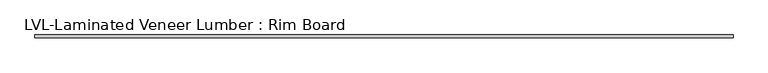
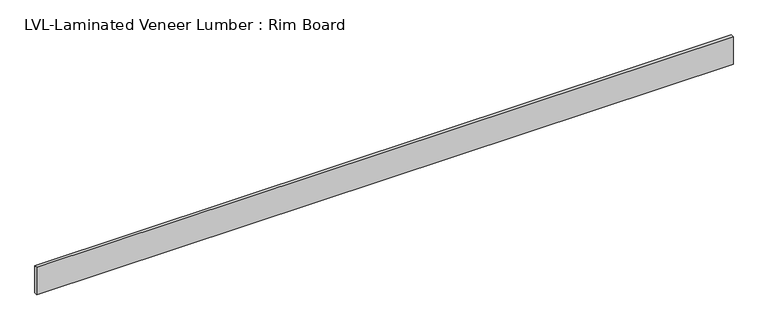
"""IFC4 building model written with IfcOpenShell, lengths in millimetres: beam geometry, LVL-Laminated Veneer Lumber : Rim Board."""

import ifcopenshell
import ifcopenshell.guid

model = None  # the IFC model being written
_history = None  # IfcOwnerHistory: only IFC2X3 demands one
_inside = {}  # id of a spatial element -> (the spatial element, [elements in it])
_under = {}  # id of a project, library or spatial element -> (it, [spatial elements below it])
_declared = {}  # id of a project -> (the project, [libraries it declares])
_typed = {}  # id of a type object -> (the type object, [elements of that type])
_made_of = {}  # id of a material, layer set ... -> (it, [elements and type objects made of it])


def new_model(schema):
    """Start an empty IFC model of exactly this schema.

    Asked for "IFC4X3", IfcOpenShell would pick the latest addendum, in which some entities
    have other attributes; the version numbers below select the first issue.
    IFC2X3 requires an IfcOwnerHistory on every rooted entity: one is made here for all.
    """
    global model, _history
    if schema == "IFC4X3":
        model = ifcopenshell.file(schema_version=(4, 3, 0, 0))
    else:
        model = ifcopenshell.file(schema=schema)
    _inside.clear()
    _under.clear()
    _declared.clear()
    _typed.clear()
    _made_of.clear()
    _history = None
    if model.schema == "IFC2X3":
        org = make("IfcOrganization", Name="unknown")
        user = make(
            "IfcPersonAndOrganization",
            ThePerson=make("IfcPerson", FamilyName="unknown"),
            TheOrganization=org,
        )
        app = make(
            "IfcApplication",
            ApplicationDeveloper=org,
            Version="unknown",
            ApplicationFullName="unknown",
            ApplicationIdentifier="unknown",
        )
        _history = make(
            "IfcOwnerHistory",
            OwningUser=user,
            OwningApplication=app,
            ChangeAction="ADDED",
            CreationDate=0,
        )
    return model


def make(cls, **values):
    """One entity of the class cls with the attributes given. An attribute that is None is left unset."""
    return model.create_entity(
        cls, **{name: value for name, value in values.items() if value is not None}
    )


def rooted(cls, **values):
    """An entity with a GlobalId (a new one), such as an element, a storey or a relation."""
    return make(cls, GlobalId=ifcopenshell.guid.new(), OwnerHistory=_history, **values)


def si_unit(unit_type, name, prefix=None):
    """IfcSIUnit, for example si_unit("LENGTHUNIT", "METRE", prefix="MILLI")."""
    return make("IfcSIUnit", UnitType=unit_type, Prefix=prefix, Name=name)


def assignment(units):
    """IfcUnitAssignment: the units of a project."""
    return None if units is None else make("IfcUnitAssignment", Units=units)


def point(xyz):
    """IfcCartesianPoint."""
    return None if xyz is None else make("IfcCartesianPoint", Coordinates=xyz)


def direction(xyz):
    """IfcDirection."""
    return None if xyz is None else make("IfcDirection", DirectionRatios=xyz)


def frame(location, z_axis=None, x_axis=None):
    """IfcAxis2Placement3D, a coordinate frame: its origin and axes. An axis left out is left unset."""
    return make(
        "IfcAxis2Placement3D",
        Location=point(location),
        Axis=direction(z_axis),
        RefDirection=direction(x_axis),
    )


def origin():
    """The frame at (0, 0, 0) with its axes left unset."""
    return frame((0.0, 0.0, 0.0))


def place(relative_to, where):
    """IfcLocalPlacement: puts the frame where relative to a parent placement (None: the world)."""
    return make(
        "IfcLocalPlacement", PlacementRelTo=relative_to, RelativePlacement=where
    )


def context(
    kind, dimensions, precision=None, world=None, true_north=None, identifier=None
):
    """IfcGeometricRepresentationContext, for example the 3D "Model" context."""
    return make(
        "IfcGeometricRepresentationContext",
        ContextIdentifier=identifier,
        ContextType=kind,
        CoordinateSpaceDimension=dimensions,
        Precision=precision,
        WorldCoordinateSystem=world,
        TrueNorth=true_north,
    )


def project(units=None, contexts=None):
    """IfcProject with its units and contexts."""
    return rooted(
        "IfcProject",
        Name="project",
        RepresentationContexts=contexts,
        UnitsInContext=assignment(units),
    )


def spatial(cls, under=None, at=None, **own):
    """A site, building, storey or space (cls), placed at a placement, below another one or the project."""
    s = rooted(cls, ObjectPlacement=at, **own)
    if under is not None:
        _under.setdefault(under.id(), (under, []))[1].append(s)
    return s


def polyline(points):
    """IfcPolyline through the points."""
    return make("IfcPolyline", Points=[point(p) for p in points])


def outline(outer, holes=None, kind="AREA"):
    """IfcArbitraryClosedProfileDef: a profile drawn as a closed curve; with holes, ...WithVoids."""
    if holes is None:
        return make("IfcArbitraryClosedProfileDef", ProfileType=kind, OuterCurve=outer)
    return make(
        "IfcArbitraryProfileDefWithVoids",
        ProfileType=kind,
        OuterCurve=outer,
        InnerCurves=holes,
    )


def extrude(swept, where, along, depth):
    """IfcExtrudedAreaSolid: the profile swept, set in the frame where, extruded along a direction by depth."""
    return make(
        "IfcExtrudedAreaSolid",
        SweptArea=swept,
        Position=where,
        ExtrudedDirection=direction(along),
        Depth=depth,
    )


def shape(context_of_items, identifier, shape_type, items):
    """IfcShapeRepresentation: the items that make up one representation, for example the "Body"."""
    return make(
        "IfcShapeRepresentation",
        ContextOfItems=context_of_items,
        RepresentationIdentifier=identifier,
        RepresentationType=shape_type,
        Items=items,
    )


def source(mapping_origin, context_of_items, identifier, shape_type, items):
    """IfcRepresentationMap: a shape defined once, which mapped items show again and again."""
    return make(
        "IfcRepresentationMap",
        MappingOrigin=mapping_origin,
        MappedRepresentation=shape(context_of_items, identifier, shape_type, items),
    )


def transform(
    local_origin,
    x_axis=None,
    y_axis=None,
    z_axis=None,
    scale=None,
    scale2=None,
    scale3=None,
    uniform=True,
):
    """IfcCartesianTransformationOperator3D, or its non-uniform kind. x_axis, y_axis, z_axis: its Axis1, 2, 3."""
    if uniform:
        return make(
            "IfcCartesianTransformationOperator3D",
            Axis1=direction(x_axis),
            Axis2=direction(y_axis),
            LocalOrigin=point(local_origin),
            Scale=scale,
            Axis3=direction(z_axis),
        )
    return make(
        "IfcCartesianTransformationOperator3DnonUniform",
        Axis1=direction(x_axis),
        Axis2=direction(y_axis),
        LocalOrigin=point(local_origin),
        Scale=scale,
        Axis3=direction(z_axis),
        Scale2=scale2,
        Scale3=scale3,
    )


def mapped(mapping_source, mapping_target):
    """IfcMappedItem: shows the shape of a source again, moved by a transform."""
    return make(
        "IfcMappedItem", MappingSource=mapping_source, MappingTarget=mapping_target
    )


def made_of(thing, what):
    """Note that an element or type object is made of a material, layer set ...; save() writes the relation."""
    if what is not None:
        _made_of.setdefault(what.id(), (what, []))[1].append(thing)
    return thing


def element(
    cls,
    number,
    at=None,
    inside=None,
    cuts=None,
    type_object=None,
    material=None,
    context=None,
    identifier="Body",
    shape_type=None,
    held_by="IfcProductDefinitionShape",
    body=None,
    shapes=None,
    **own,
):
    """One element of the class cls, such as IfcWall. Its Tag is "e" and its number.

    at: its placement. inside: the storey or other place that contains it. cuts: it is an
    opening in that element (IfcRelVoidsElement). A single representation is given by context,
    identifier, shape_type and body (its items); several are given by shapes. held_by: the class
    of the entity that holds the representations. save() writes the other relations.
    """
    e = rooted(cls, Tag="e%d" % number, ObjectPlacement=at, **own)
    if body is not None:
        shapes = [shape(context, identifier, shape_type, body)]
    if shapes is not None:
        e.Representation = make(held_by, Representations=shapes)
    if inside is not None:
        _inside.setdefault(inside.id(), (inside, []))[1].append(e)
    if cuts is not None:
        rooted(
            "IfcRelVoidsElement", RelatingBuildingElement=cuts, RelatedOpeningElement=e
        )
    if type_object is not None:
        _typed.setdefault(type_object.id(), (type_object, []))[1].append(e)
    return made_of(e, material)


def aggregate(whole, parts):
    """IfcRelAggregates: a whole, such as a stair, and the parts it consists of."""
    return rooted("IfcRelAggregates", RelatingObject=whole, RelatedObjects=parts)


def save(model, path):
    """Write the relations noted so far, then the file.

    IfcRelAggregates (storeys below a building ...), IfcRelContainedInSpatialStructure (elements
    in a storey), IfcRelDefinesByType, IfcRelAssociatesMaterial and IfcRelDeclares: one each for
    every whole, place, type object, material and project.
    """
    for whole, parts in _under.values():
        aggregate(whole, parts)
    for where, things in _inside.values():
        rooted(
            "IfcRelContainedInSpatialStructure",
            RelatedElements=things,
            RelatingStructure=where,
        )
    for kind, things in _typed.values():
        rooted("IfcRelDefinesByType", RelatedObjects=things, RelatingType=kind)
    for what, things in _made_of.values():
        rooted("IfcRelAssociatesMaterial", RelatedObjects=things, RelatingMaterial=what)
    for by, libraries in _declared.values():
        rooted("IfcRelDeclares", RelatingContext=by, RelatedDefinitions=libraries)
    model.write(path)


def lvl_laminated_veneer_lumber_rim_board_7eb16bd1(model_context):
    return source(origin(), model_context, "Body", "SweptSolid", [
        extrude(outline(polyline([(6406.35625, 15.875), (6406.35625, -15.875), (-840.58125, -15.875), (-840.58125, 15.875), (6406.35625, 15.875)])), frame((0.0, 0.0, -150.8125), z_axis=(0.0, 0.0, 1.0), x_axis=(1.0, 0.0, 0.0)), (0.0, 0.0, 1.0), 301.625),
    ])


if __name__ == "__main__":
    model = new_model("IFC4")
    model_context = context("Model", 3, world=origin())
    ifc_project = project(units=[si_unit("LENGTHUNIT", "METRE", prefix="MILLI")], contexts=[model_context])
    site = spatial("IfcSite", under=ifc_project)
    building = spatial("IfcBuilding", under=site)
    placement = place(None, origin())
    lvl_laminated_veneer_lumber_rim_board_shape = lvl_laminated_veneer_lumber_rim_board_7eb16bd1(model_context)
    element("IfcBeam", 1, ObjectType="LVL-Laminated Veneer Lumber : Rim Board", at=placement, inside=building, context=model_context, shape_type="MappedRepresentation", body=[
        mapped(lvl_laminated_veneer_lumber_rim_board_shape, transform((0.0, 0.0, 0.0), x_axis=(1.0, 0.0, 0.0), y_axis=(0.0, 1.0, 0.0), z_axis=(0.0, 0.0, 1.0))),
    ])
    save(model, "model.ifc")

# Revit data of these elements
# Type "LVL-Laminated Veneer Lumber : Rim Board"
#   Assembly Code = "B10"
#   Cost = 4.6
#   Length [instance default] = 5' - 0"
#   b = 0' - 1 1/4"
#   d = 0' - 11 7/8"
#   Structural Material [instance default] = Softwood, Lumber
# Element 1 (IfcBeam, "LVL-Laminated Veneer Lumber : Rim Board")
#   Structural Material = Douglas Fir #2
#   Materials on its faces: "Douglas Fir #2"
# Materials
#   "Softwood, Lumber": class "Wood", colour RGB 223 192 134, transparency 0, Description = "Pinus Echinata", Cost = 0
#   "Douglas Fir #2": class "Wood", colour RGB 223 192 134, transparency 0, Description = "Pinus Echinata", Cost = 0
